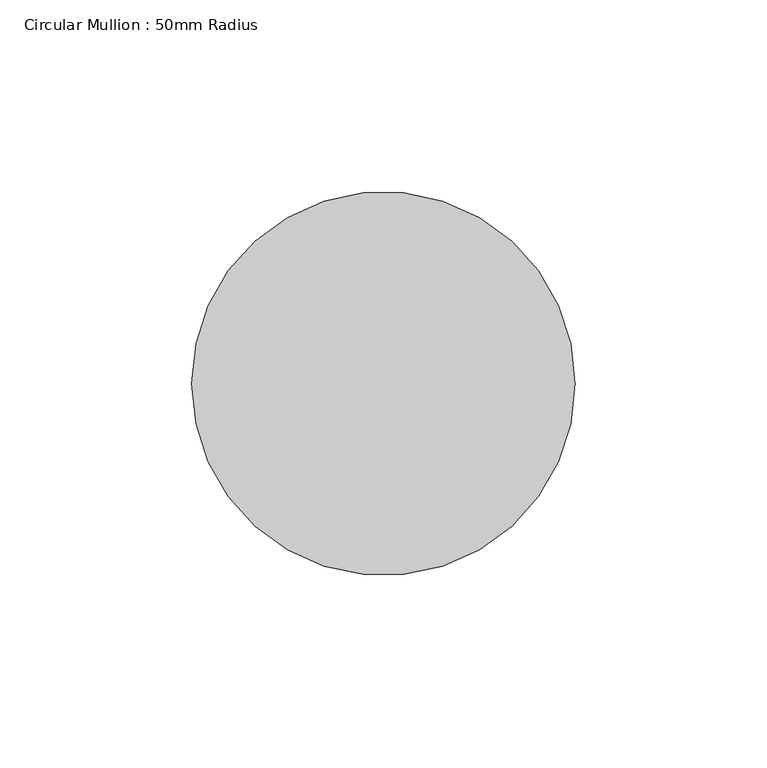
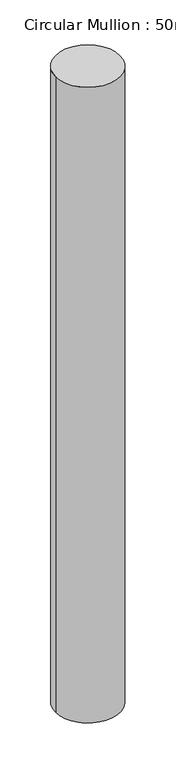
"""IFC4 building model written with IfcOpenShell, lengths in millimetres: member geometry, Circular Mullion : 50mm Radius."""

from ifc_helpers import new_model, si_unit, point, frame, origin, origin_2d, place, context, project, spatial, circle_curve, trimmed, segment, composite_curve, outline, extrude, source, transform, mapped, element, save


def circular_mullion_50mm_radius_7aba59ff(model_context):
    return source(origin(), model_context, "Body", "SweptSolid", [
        extrude(outline(composite_curve([segment(trimmed(circle_curve(origin_2d(), 50.0), [point((50.0, 0.0))], [point((-50.0, 0.0))], False, "CARTESIAN"), True, "CONTINUOUS"), segment(trimmed(circle_curve(origin_2d(), 50.0), [point((-50.0, 0.0))], [point((50.0, 0.0))], False, "CARTESIAN"), True, "CONTINUOUS")], self_intersect=False)), frame((0.0, 0.0, -1046.0523821), z_axis=(0.0, 0.0, 1.0), x_axis=(1.0, 0.0, 0.0)), (0.0, 0.0, 1.0), 1046.0523821),
    ])


if __name__ == "__main__":
    model = new_model("IFC4")
    model_context = context("Model", 3, world=origin())
    ifc_project = project(units=[si_unit("LENGTHUNIT", "METRE", prefix="MILLI")], contexts=[model_context])
    site = spatial("IfcSite", under=ifc_project)
    building = spatial("IfcBuilding", under=site)
    placement = place(None, origin())
    circular_mullion_50mm_radius_shape = circular_mullion_50mm_radius_7aba59ff(model_context)
    element("IfcMember", 1, ObjectType="Circular Mullion : 50mm Radius", at=placement, inside=building, context=model_context, shape_type="MappedRepresentation", body=[
        mapped(circular_mullion_50mm_radius_shape, transform((0.0, 0.0, 0.0), x_axis=(1.0, 0.0, 0.0), y_axis=(0.0, 1.0, 0.0), z_axis=(0.0, 0.0, 1.0))),
    ])
    save(model, "model.ifc")

# Revit data of these elements
# Type "Circular Mullion : 50mm Radius"
#   built-in parameter 1007350 = 0.164042 (stored number, unit not read)
# Element 1 (IfcMember, "Circular Mullion : 50mm Radius")
#   Materials on its faces: "Aluminium"
# Materials
#   "Aluminium": class "Metal", colour RGB 247 247 247, transparency 0, Description = "Aluminium 6061", Cost = 0
